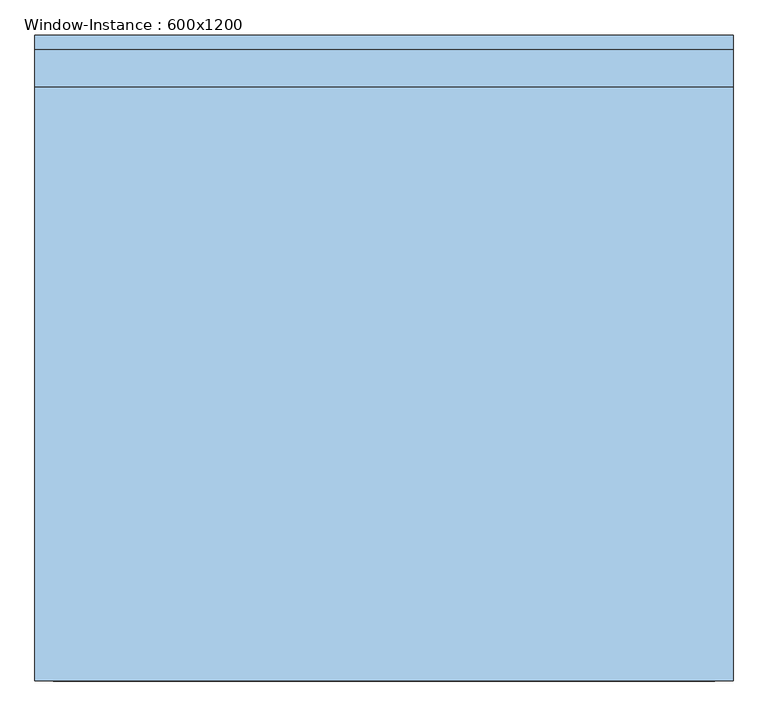
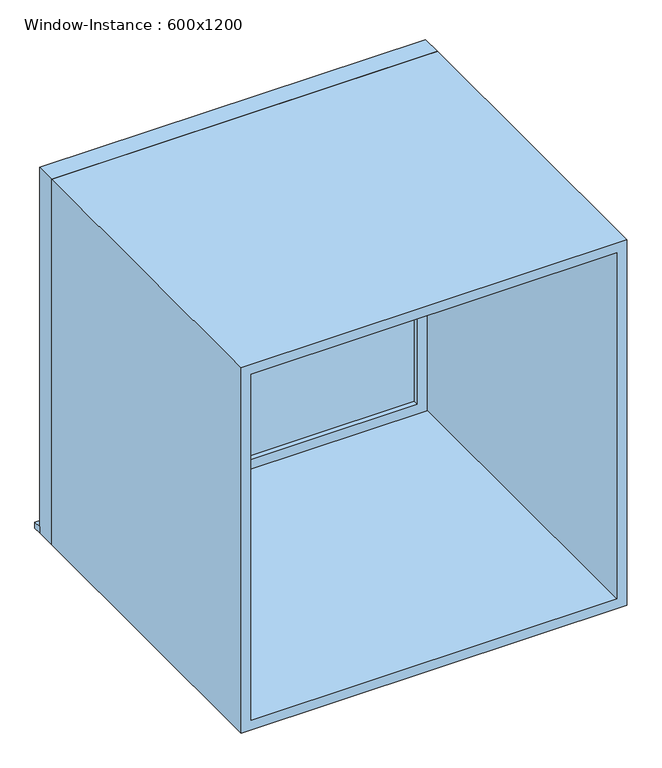
"""IFC4 building model written with IfcOpenShell, lengths in millimetres: window geometry, Window-Instance : 600x1200."""

from ifc_helpers import new_model, si_unit, frame, origin, place, context, project, spatial, polyline, outline, extrude, source, transform, mapped, element, save


def window_instance_600x1200_b5ab94bb(model_context):
    return source(origin(), model_context, "Body", "SweptSolid", [
        extrude(outline(polyline([(-638.1, 567.9), (561.9, 567.9), (561.9, 542.5), (-638.1, 542.5), (-638.1, 567.9)])), frame((0.0, 0.0, 900.0), z_axis=(0.0, 0.0, 1.0), x_axis=(1.0, 0.0, 0.0)), (0.0, 0.0, 1.0), 19.05),
        extrude(outline(polyline([(498.4, 493.925), (-574.6, 493.925), (-574.6, 506.625), (498.4, 506.625), (498.4, 493.925)])), frame((0.0, 0.0, 963.5), z_axis=(0.0, 0.0, 1.0), x_axis=(1.0, 0.0, 0.0)), (0.0, 0.0, 1.0), 1073.0),
        extrude(outline(polyline([(2080.95, -619.05), (919.05, -619.05), (919.05, 542.85), (2080.95, 542.85), (2080.95, -619.05)]), holes=[polyline([(2036.5, -574.6), (2036.5, 498.4), (963.5, 498.4), (963.5, -574.6), (2036.5, -574.6)])]), frame((0.0, 478.05, 0.0), z_axis=(0.0, 1.0, 0.0), x_axis=(0.0, 0.0, 1.0)), (0.0, 0.0, 1.0), 44.45),
        extrude(outline(polyline([(2100.0, -638.1), (900.0, -638.1), (900.0, 561.9), (2100.0, 561.9), (2100.0, -638.1)]), holes=[polyline([(2068.25, -606.35), (2068.25, 530.15), (931.75, 530.15), (931.75, -606.35), (2068.25, -606.35)])]), frame((0.0, -542.5, 0.0), z_axis=(0.0, 1.0, 0.0), x_axis=(0.0, 0.0, 1.0)), (0.0, 0.0, 1.0), 1020.55),
        extrude(outline(polyline([(2100.0, 561.9), (2100.0, -638.1), (900.0, -638.1), (900.0, 561.9), (2100.0, 561.9)]), holes=[polyline([(2080.95, 542.85), (919.05, 542.85), (919.05, -619.05), (2080.95, -619.05), (2080.95, 542.85)])]), frame((0.0, 478.05, 0.0), z_axis=(0.0, 1.0, 0.0), x_axis=(0.0, 0.0, 1.0)), (0.0, 0.0, 1.0), 64.45),
    ])


if __name__ == "__main__":
    model = new_model("IFC4")
    model_context = context("Model", 3, world=origin())
    ifc_project = project(units=[si_unit("LENGTHUNIT", "METRE", prefix="MILLI")], contexts=[model_context])
    site = spatial("IfcSite", under=ifc_project)
    building = spatial("IfcBuilding", under=site)
    placement = place(None, origin())
    window_instance_600x1200_shape = window_instance_600x1200_b5ab94bb(model_context)
    element("IfcWindow", 1, ObjectType="Window-Instance : 600x1200", at=placement, inside=building, context=model_context, shape_type="MappedRepresentation", body=[
        mapped(window_instance_600x1200_shape, transform((0.0, 0.0, 0.0), x_axis=(1.0, 0.0, 0.0), y_axis=(0.0, 1.0, 0.0), z_axis=(0.0, 0.0, 1.0))),
    ])
    save(model, "model.ifc")

# Revit data of these elements
# Type "Window-Instance : 600x1200"
#   Type Mark = "7"
#   Construction Type Id = "GSP4R"
#   Assembly Code = "B2020100"
#   Analytic Construction = "1/8 in Pilkington single glazing"
#   Visual Light Transmittance = 0.9
#   Thermal Resistance (R) = 0.149095 (m²·K)/W
#   Solar Heat Gain Coefficient = 0.86
#   Heat Transfer Coefficient (U) = 6.70716 W/(m²·K)
#   Height [instance default] = 1200 mm
#   Default Sill Height = 900 mm
#   Width [instance default] = 600 mm
#   Window Inset = 20 mm
#   Glass Pane Material = WW-EC-GL-Storefront
#   Sash Material = WW-EC-RGB-White
#   Wall Closure = (empty or 0)
# Element 1 (IfcWindow, "Window-Instance : 600x1200")
#   Width = 1200 mm
#   Materials on its faces: "WW-EC-RGB-White", "WW-EC-GL-Storefront"
# Materials
#   "WW-EC-GL-Storefront": class "Glass", colour RGB 236 240 239, transparency 0.85, Description = "Storefront Glass", Cost = 0
#   "WW-EC-RGB-White": class "Generic", colour RGB 255 255 255, transparency 0, Comments = "If region requests off-white, swith asset color to RGB 231-228-220", Description = "Generic Color", Cost = 0
